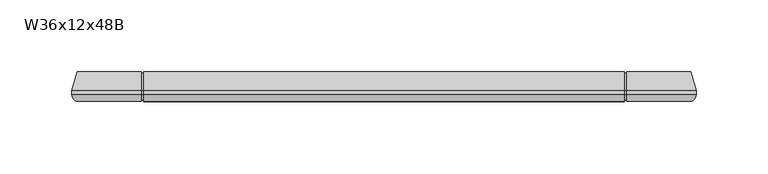
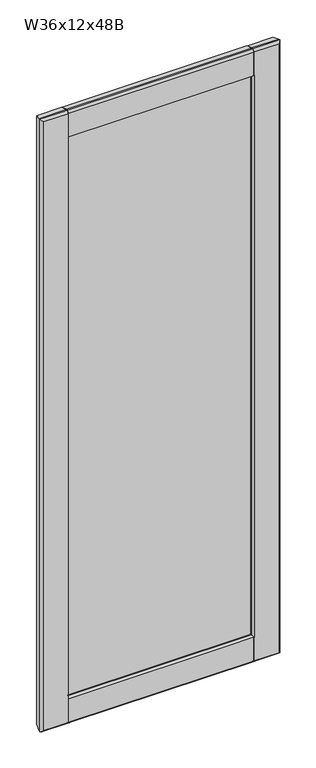
"""IFC4 building model written with IfcOpenShell, lengths in millimetres: furniture geometry, Cabinet-Wall-Merillat-Double_Door-Marlin : W36x12x48B."""

from ifc_helpers import new_model, si_unit, frame, origin, place, context, project, spatial, polyline, circle_curve, ellipse_curve, outline, extrude, source, transform, mapped, element, save
from ifc_brep_helpers import plane_surface, cylinder_surface, advanced_brep


def w36x12x48b_c809501e(model_context):
    return source(origin(), model_context, "Body", "SolidModel", [
        advanced_brep(
        [(541.0528392, -401.6121, 2108.2), (537.9563467, -406.0825, 2105.1035075), (537.9563467, -406.0825, 942.8964925), (541.0528392, -401.6121, 939.8), (541.0528392, -398.8435, 939.8), (541.0528392, -398.8435, 2108.2), (537.5476392, -385.7625, 943.3052), (537.5476392, -385.7625, 2104.6948), (492.8516765, -385.7625, 2059.9988372), (492.8516765, -385.7625, 988.0011628), (492.4815448, -386.55625, 988.3712945), (490.4003857, -391.01931, 990.4524535), (490.4003857, -391.01931, 2057.5475465), (492.4815448, -386.55625, 2059.6287055), (491.8001552, -393.2594093, 989.052684), (491.8001552, -393.2594093, 2058.947316), (506.1278392, -393.5095, 974.725), (506.1278392, -393.5095, 2073.275), (506.1278392, -398.3355, 974.725), (506.1278392, -398.3355, 2073.275), (491.8001552, -398.5855907, 989.052684), (491.8001552, -398.5855907, 2058.947316), (490.4003857, -400.82569, 990.4524535), (490.4003857, -400.82569, 2057.5475465), (492.4815448, -405.28875, 988.3712945), (492.848809, -406.0763508, 988.0040302), (492.8516765, -406.0825, 2059.9988372), (492.4815448, -405.28875, 2059.6287055), (492.848809, -406.0825, 942.8964925), (492.848809, -401.6121, 939.8), (110.7618317, -406.0825, 942.8964925), (107.6653392, -401.6121, 939.8), (155.8295579, -401.6121, 939.8), (155.8295579, -406.0825, 942.8964925), (491.261309, -401.6121, 939.8), (491.261309, -406.0825, 942.8964925), (157.4170579, -406.0825, 942.8964925), (157.4170579, -401.6121, 939.8), (492.848809, -398.8435, 939.8), (107.6653392, -398.8435, 939.8), (155.8295579, -398.8435, 939.8), (491.261309, -398.8435, 939.8), (157.4170579, -398.8435, 939.8), (492.848809, -385.7625, 943.3052), (111.1705392, -385.7625, 943.3052), (155.8295579, -385.7625, 943.3052), (491.261309, -385.7625, 943.3052), (157.4170579, -385.7625, 943.3052), (158.3177927, -391.01931, 990.4524535), (491.261309, -386.55625, 988.3712945), (491.261309, -385.7625, 988.0011628), (157.4170579, -385.7625, 988.0011628), (157.4170579, -386.55625, 988.3712945), (156.2366337, -386.55625, 988.3712945), (156.9180233, -393.2594093, 989.052684), (142.5903392, -393.5095, 974.725), (142.5903392, -398.3355, 974.725), (156.9180233, -398.5855907, 989.052684), (158.3177927, -400.82569, 990.4524535), (156.2366337, -405.28875, 988.3712945), (157.4170579, -405.28875, 988.3712945), (157.4170579, -406.0825, 988.0011628), (491.261309, -406.0825, 988.0011628), (491.261309, -405.28875, 988.3712945), (110.7618317, -406.0825, 2105.1035075), (107.6653392, -401.6121, 2108.2), (107.6653392, -398.8435, 2108.2), (111.1705392, -385.7625, 2104.6948), (155.866502, -385.7625, 988.0011628), (155.866502, -385.7625, 2059.9988372), (156.2366337, -386.55625, 2059.6287055), (158.3177927, -391.01931, 2057.5475465), (156.9180233, -393.2594093, 2058.947316), (142.5903392, -393.5095, 2073.275), (142.5903392, -398.3355, 2073.275), (156.9180233, -398.5855907, 2058.947316), (158.3177927, -400.82569, 2057.5475465), (156.2366337, -405.28875, 2059.6287055), (155.866502, -406.0825, 2059.9988372), (155.866502, -406.0825, 988.0011628), (155.8295579, -406.0825, 2105.1035075), (155.8295579, -401.6121, 2108.2), (492.848809, -401.6121, 2108.2), (492.848809, -406.0825, 2105.1035075), (157.4170579, -401.6121, 2108.2), (157.4170579, -406.0825, 2105.1035075), (491.261309, -406.0825, 2105.1035075), (491.261309, -401.6121, 2108.2), (155.8295579, -398.8435, 2108.2), (492.848809, -398.8435, 2108.2), (157.4170579, -398.8435, 2108.2), (491.261309, -398.8435, 2108.2), (155.8295579, -385.7625, 2104.6948), (492.848809, -385.7625, 2104.6948), (157.4170579, -385.7625, 2104.6948), (491.261309, -385.7625, 2104.6948), (157.4170579, -385.7625, 2059.9988372), (491.261309, -385.7625, 2059.9988372), (157.4170579, -386.55625, 2059.6287055), (491.261309, -386.55625, 2059.6287055), (491.261309, -405.28875, 2059.6287055), (491.261309, -406.0825, 2059.9988372), (157.4170579, -406.0825, 2059.9988372), (157.4170579, -405.28875, 2059.6287055), (157.4170579, -386.55625, 2104.0857412), (157.4170579, -398.9480037, 2107.40625), (157.4170579, -401.6121, 2107.40625), (157.4170579, -405.28875, 2104.9526052), (155.8295579, -405.28875, 2059.6287055), (155.8295579, -405.28875, 2104.9526052), (155.8295579, -401.6121, 2107.40625), (155.8295579, -398.9480037, 2107.40625), (155.8295579, -386.55625, 2104.0857412), (155.8295579, -386.55625, 2059.6287055), (492.848809, -386.55625, 2059.6287055), (492.848809, -386.55625, 2104.0857412), (492.848809, -398.9480037, 2107.40625), (492.848809, -401.6121, 2107.40625), (492.848809, -405.28875, 2104.9526052), (492.848809, -405.28875, 2059.6287055), (491.261309, -405.28875, 2104.9526052), (491.261309, -401.6121, 2107.40625), (491.261309, -398.9480037, 2107.40625), (491.261309, -386.55625, 2104.0857412), (492.848809, -405.28875, 988.3712945), (492.848809, -405.28875, 943.0473948), (492.848809, -401.6121, 940.59375), (492.848809, -398.9480037, 940.59375), (492.848809, -386.55625, 943.9142588), (492.848809, -386.55625, 988.3712945), (491.261309, -386.55625, 943.9142588), (491.261309, -398.9480037, 940.59375), (491.261309, -401.6121, 940.59375), (491.261309, -405.28875, 943.0473948), (157.4170579, -405.28875, 943.0473948), (157.4170579, -401.6121, 940.59375), (157.4170579, -398.9480037, 940.59375), (157.4170579, -386.55625, 943.9142588), (155.8295579, -405.28875, 988.3712945), (155.8295579, -386.55625, 988.3712945), (155.8295579, -386.55625, 943.9142588), (155.8295579, -398.9480037, 940.59375), (155.8295579, -401.6121, 940.59375), (155.8295579, -405.28875, 943.0473948)],
        [
            (0, 1, ellipse_curve(frame((536.2776392, -401.6121, 2103.4248), z_axis=(0.7071067811865475, 0.0, -0.7071067811865475), x_axis=(0.7071067811865474, 0.0, 0.7071067811865476)), 6.7531526, 4.7752)),
            (1, 2),
            (2, 3, ellipse_curve(frame((536.2776392, -401.6121, 944.5752), z_axis=(0.7071067811865475, 0.0, 0.7071067811865475), x_axis=(-0.7071067811865474, 0.0, 0.7071067811865476)), 6.7531526, 4.7752)),
            (3, 0),
            (3, 4),
            (4, 5),
            (5, 0),
            (4, 6),
            (6, 7),
            (7, 5),
            (8, 9),
            (9, 10),
            (10, 11),
            (11, 12),
            (12, 13),
            (13, 8),
            (11, 14, ellipse_curve(frame((491.8276392, -391.6848492, 989.0252), z_axis=(0.7071067811865475, 0.0, 0.7071067811865475), x_axis=(-0.7071067811865474, 0.0, 0.7071067811865476)), 2.2271035, 1.5748)),
            (14, 15),
            (15, 12, ellipse_curve(frame((491.8276392, -391.6848492, 2058.9748), z_axis=(0.7071067811865475, 0.0, -0.7071067811865475), x_axis=(0.7071067811865474, 0.0, 0.7071067811865476)), 2.2271035, 1.5748)),
            (14, 16),
            (16, 17),
            (17, 15),
            (16, 18),
            (18, 19),
            (19, 17),
            (18, 20),
            (20, 21),
            (21, 19),
            (20, 22, ellipse_curve(frame((491.8276392, -400.1601508, 989.0252), z_axis=(0.7071067811865475, 0.0, 0.7071067811865475), x_axis=(-0.7071067811865474, 0.0, 0.7071067811865476)), 2.2271035, 1.5748)),
            (22, 23),
            (23, 21, ellipse_curve(frame((491.8276392, -400.1601508, 2058.9748), z_axis=(0.7071067811865475, 0.0, -0.7071067811865475), x_axis=(0.7071067811865474, 0.0, 0.7071067811865476)), 2.2271035, 1.5748)),
            (22, 24),
            (24, 25),
            (25, 26),
            (26, 27),
            (27, 23),
            (2, 28),
            (28, 29, circle_curve(frame((492.848809, -401.6121, 944.5752), z_axis=(1.0, 0.0, 0.0), x_axis=(0.0, 1.0, 0.0)), 4.7752)),
            (29, 3),
            (30, 31, ellipse_curve(frame((112.4405392, -401.6121, 944.5752), z_axis=(0.7071067811865475, 0.0, -0.7071067811865475), x_axis=(0.7071067811865476, 0.0, 0.7071067811865474)), 6.7531526, 4.7752)),
            (31, 32),
            (32, 33, circle_curve(frame((155.8295579, -401.6121, 944.5752), z_axis=(-1.0, 0.0, 0.0), x_axis=(0.0, 1.0, 0.0)), 4.7752)),
            (33, 30),
            (34, 35, circle_curve(frame((491.261309, -401.6121, 944.5752), z_axis=(-1.0, 0.0, 0.0), x_axis=(0.0, 1.0, 0.0)), 4.7752)),
            (35, 36),
            (36, 37, circle_curve(frame((157.4170579, -401.6121, 944.5752), z_axis=(1.0, 0.0, 0.0), x_axis=(0.0, 1.0, 0.0)), 4.7752)),
            (37, 34),
            (29, 38),
            (38, 4),
            (31, 39),
            (39, 40),
            (40, 32),
            (41, 34),
            (37, 42),
            (42, 41),
            (38, 43),
            (43, 6),
            (39, 44),
            (44, 45),
            (45, 40),
            (46, 41),
            (42, 47),
            (47, 46),
            (48, 11),
            (10, 49),
            (49, 50),
            (50, 51),
            (51, 52),
            (52, 53),
            (53, 48),
            (48, 54, ellipse_curve(frame((156.8905392, -391.6848492, 989.0252), z_axis=(0.7071067811865475, 0.0, -0.7071067811865475), x_axis=(0.7071067811865476, 0.0, 0.7071067811865474)), 2.2271035, 1.5748)),
            (54, 14),
            (54, 55),
            (55, 16),
            (55, 56),
            (56, 18),
            (56, 57),
            (57, 20),
            (57, 58, ellipse_curve(frame((156.8905392, -400.1601508, 989.0252), z_axis=(0.7071067811865475, 0.0, -0.7071067811865475), x_axis=(0.7071067811865476, 0.0, 0.7071067811865474)), 2.2271035, 1.5748)),
            (58, 22),
            (58, 59),
            (59, 60),
            (60, 61),
            (61, 62),
            (62, 63),
            (63, 24),
            (30, 64),
            (64, 65, ellipse_curve(frame((112.4405392, -401.6121, 2103.4248), z_axis=(-0.7071067811865475, 0.0, -0.7071067811865475), x_axis=(0.7071067811865474, 0.0, -0.7071067811865476)), 6.7531526, 4.7752)),
            (65, 31),
            (65, 66),
            (66, 39),
            (66, 67),
            (67, 44),
            (68, 69),
            (69, 70),
            (70, 71),
            (71, 48),
            (53, 68),
            (71, 72, ellipse_curve(frame((156.8905392, -391.6848492, 2058.9748), z_axis=(-0.7071067811865475, 0.0, -0.7071067811865475), x_axis=(0.7071067811865474, 0.0, -0.7071067811865476)), 2.2271035, 1.5748)),
            (72, 54),
            (72, 73),
            (73, 55),
            (73, 74),
            (74, 56),
            (74, 75),
            (75, 57),
            (75, 76, ellipse_curve(frame((156.8905392, -400.1601508, 2058.9748), z_axis=(-0.7071067811865475, 0.0, -0.7071067811865475), x_axis=(0.7071067811865474, 0.0, -0.7071067811865476)), 2.2271035, 1.5748)),
            (76, 58),
            (76, 77),
            (77, 78),
            (78, 79),
            (79, 59),
            (64, 80),
            (80, 81, circle_curve(frame((155.8295579, -401.6121, 2103.4248), z_axis=(-1.0, 0.0, 0.0), x_axis=(0.0, 1.0, 0.0)), 4.7752)),
            (81, 65),
            (0, 82),
            (82, 83, circle_curve(frame((492.848809, -401.6121, 2103.4248), z_axis=(1.0, 0.0, 0.0), x_axis=(0.0, 1.0, 0.0)), 4.7752)),
            (83, 1),
            (84, 85, circle_curve(frame((157.4170579, -401.6121, 2103.4248), z_axis=(1.0, 0.0, 0.0), x_axis=(0.0, 1.0, 0.0)), 4.7752)),
            (85, 86),
            (86, 87, circle_curve(frame((491.261309, -401.6121, 2103.4248), z_axis=(-1.0, 0.0, 0.0), x_axis=(0.0, 1.0, 0.0)), 4.7752)),
            (87, 84),
            (81, 88),
            (88, 66),
            (5, 89),
            (89, 82),
            (90, 84),
            (87, 91),
            (91, 90),
            (88, 92),
            (92, 67),
            (7, 93),
            (93, 89),
            (94, 90),
            (91, 95),
            (95, 94),
            (92, 69),
            (68, 45),
            (50, 46),
            (47, 51),
            (43, 9),
            (8, 93),
            (96, 94),
            (95, 97),
            (97, 96),
            (12, 71),
            (70, 98),
            (98, 96),
            (97, 99),
            (99, 13),
            (15, 72),
            (17, 73),
            (19, 74),
            (21, 75),
            (23, 76),
            (27, 100),
            (100, 101),
            (101, 102),
            (102, 103),
            (103, 77),
            (83, 26),
            (25, 28),
            (33, 79),
            (78, 80),
            (35, 62),
            (61, 36),
            (85, 102),
            (101, 86),
            (98, 104),
            (104, 105),
            (105, 106),
            (106, 107, circle_curve(frame((157.4170579, -401.6121, 2103.4248), z_axis=(1.0, 0.0, 0.0), x_axis=(0.0, 0.0, 1.0)), 3.98145)),
            (107, 103),
            (78, 108),
            (108, 109),
            (109, 110, circle_curve(frame((155.8295579, -401.6121, 2103.4248), z_axis=(-1.0, 0.0, 0.0), x_axis=(0.0, 0.0, 1.0)), 3.98145)),
            (110, 111),
            (111, 112),
            (112, 113),
            (113, 69),
            (77, 108),
            (107, 109),
            (106, 110),
            (105, 111),
            (104, 112),
            (70, 113),
            (8, 114),
            (114, 115),
            (115, 116),
            (116, 117),
            (117, 118, circle_curve(frame((492.848809, -401.6121, 2103.4248), z_axis=(1.0, 0.0, 0.0), x_axis=(0.0, 0.0, 1.0)), 3.98145)),
            (118, 119),
            (119, 26),
            (100, 120),
            (120, 121, circle_curve(frame((491.261309, -401.6121, 2103.4248), z_axis=(-1.0, 0.0, 0.0), x_axis=(0.0, 0.0, 1.0)), 3.98145)),
            (121, 122),
            (122, 123),
            (123, 99),
            (119, 27),
            (118, 120),
            (117, 121),
            (116, 122),
            (115, 123),
            (114, 13),
            (25, 124),
            (124, 125),
            (125, 126, circle_curve(frame((492.848809, -401.6121, 944.5752), z_axis=(1.0, 0.0, 0.0), x_axis=(0.0, 0.0, 1.0)), 3.98145)),
            (126, 127),
            (127, 128),
            (128, 129),
            (129, 9),
            (49, 130),
            (130, 131),
            (131, 132),
            (132, 133, circle_curve(frame((491.261309, -401.6121, 944.5752), z_axis=(-1.0, 0.0, 0.0), x_axis=(0.0, 0.0, 1.0)), 3.98145)),
            (133, 63),
            (129, 10),
            (128, 130),
            (127, 131),
            (126, 132),
            (125, 133),
            (124, 24),
            (60, 134),
            (134, 135, circle_curve(frame((157.4170579, -401.6121, 944.5752), z_axis=(1.0, 0.0, 0.0), x_axis=(0.0, 0.0, 1.0)), 3.98145)),
            (135, 136),
            (136, 137),
            (137, 52),
            (138, 79),
            (68, 139),
            (139, 140),
            (140, 141),
            (141, 142),
            (142, 143, circle_curve(frame((155.8295579, -401.6121, 944.5752), z_axis=(-1.0, 0.0, 0.0), x_axis=(0.0, 0.0, 1.0)), 3.98145)),
            (143, 138),
            (138, 59),
            (53, 139),
            (137, 140),
            (136, 141),
            (135, 142),
            (134, 143),
        ],
        [
            cylinder_surface(frame((536.2776392, -401.6121, 2108.2), z_axis=(0.0, 0.0, 1.0), x_axis=(0.0, 1.0, 0.0)), 4.7752),
            plane_surface(frame((541.0528392, -401.6121, 2108.2), z_axis=(1.0, 0.0, 0.0), x_axis=(0.0, 0.0, -1.0))),
            plane_surface(frame((541.0528392, -398.8435, 2108.2), z_axis=(0.9659229350723619, 0.25882983502910506, 0.0), x_axis=(0.0, 0.0, -1.0))),
            plane_surface(frame((492.8516765, -385.7625, 2059.9988372), z_axis=(-0.9063077870366099, 0.4226182617407856, 0.0), x_axis=(0.0, 0.0, -1.0))),
            cylinder_surface(frame((491.8276392, -391.6848492, 2108.2), z_axis=(0.0, 0.0, 1.0000000000000002), x_axis=(-0.01745240643729364, -0.9998476951563912, 0.0)), 1.5748),
            plane_surface(frame((491.8001552, -393.2594093, 2058.947316), z_axis=(-0.017452406437322144, -0.9998476951563906, 0.0), x_axis=(0.0, 0.0, -1.0))),
            plane_surface(frame((506.1278392, -393.5095, 2073.275), z_axis=(-1.0, 0.0, 0.0), x_axis=(0.0, 0.0, -1.0))),
            plane_surface(frame((506.1278392, -398.3355, 2073.275), z_axis=(-0.01745240643727848, 0.9998476951563914, 0.0), x_axis=(0.0, 0.0, -1.0))),
            cylinder_surface(frame((491.8276392, -400.1601508, 2108.2), z_axis=(0.0, 0.0, 1.0000000000000002), x_axis=(-0.9063077870367326, -0.42261826174052236, 0.0)), 1.5748),
            plane_surface(frame((490.4003857, -400.82569, 2057.5475465), z_axis=(-0.9063077870366333, -0.4226182617407352, 0.0), x_axis=(0.0, 0.0, -1.0))),
            cylinder_surface(frame((541.0528392, -401.6121, 944.5752), z_axis=(1.0, 0.0, 0.0), x_axis=(0.0, 1.0, 0.0)), 4.7752),
            plane_surface(frame((541.0528392, -401.6121, 939.8), z_axis=(0.0, 0.0, -1.0), x_axis=(-1.0, 0.0, 0.0))),
            plane_surface(frame((541.0528392, -398.8435, 939.8), z_axis=(0.0, 0.2588298350291095, -0.9659229350723607), x_axis=(-1.0, 0.0, 0.0))),
            plane_surface(frame((492.8516765, -385.7625, 988.0011628), z_axis=(0.0, 0.42261826174078143, 0.9063077870366119), x_axis=(-1.0, 0.0, 0.0))),
            cylinder_surface(frame((541.0528392, -391.6848492, 989.0252), z_axis=(1.0000000000000002, 0.0, 0.0), x_axis=(0.0, -0.9998476951563913, 0.017452406437289025)), 1.5748),
            plane_surface(frame((491.8001552, -393.2594093, 989.052684), z_axis=(0.0, -0.9998476951563907, 0.01745240643731753), x_axis=(-1.0, 0.0, 0.0))),
            plane_surface(frame((506.1278392, -393.5095, 974.725), z_axis=(0.0, 0.0, 1.0), x_axis=(-1.0, 0.0, 0.0))),
            plane_surface(frame((506.1278392, -398.3355, 974.725), z_axis=(0.0, 0.9998476951563913, 0.017452406437283095), x_axis=(-1.0, 0.0, 0.0))),
            cylinder_surface(frame((541.0528392, -400.1601508, 989.0252), z_axis=(1.0000000000000002, 0.0, 0.0), x_axis=(0.0, -0.4226182617405265, 0.9063077870367306)), 1.5748),
            plane_surface(frame((490.4003857, -400.82569, 990.4524535), z_axis=(0.0, -0.4226182617407394, 0.9063077870366314), x_axis=(-1.0, 0.0, 0.0))),
            cylinder_surface(frame((112.4405392, -401.6121, 939.8), z_axis=(0.0, 0.0, -1.0), x_axis=(0.0, 1.0, 0.0)), 4.7752),
            plane_surface(frame((107.6653392, -401.6121, 939.8), z_axis=(-1.0, 0.0, 0.0), x_axis=(0.0, 0.0, 1.0))),
            plane_surface(frame((107.6653392, -398.8435, 939.8), z_axis=(-0.9659229350723619, 0.25882983502910506, 0.0), x_axis=(0.0, 0.0, 1.0))),
            plane_surface(frame((155.866502, -385.7625, 988.0011628), z_axis=(0.9063077870366099, 0.4226182617407856, 0.0), x_axis=(0.0, 0.0, 1.0))),
            cylinder_surface(frame((156.8905392, -391.6848492, 939.8), z_axis=(0.0, 0.0, -1.0000000000000002), x_axis=(0.01745240643729364, -0.9998476951563912, 0.0)), 1.5748),
            plane_surface(frame((156.9180233, -393.2594093, 989.052684), z_axis=(0.017452406437322144, -0.9998476951563906, 0.0), x_axis=(0.0, 0.0, 1.0))),
            plane_surface(frame((142.5903392, -393.5095, 974.725), z_axis=(1.0, 0.0, 0.0), x_axis=(0.0, 0.0, 1.0))),
            plane_surface(frame((142.5903392, -398.3355, 974.725), z_axis=(0.01745240643727848, 0.9998476951563914, 0.0), x_axis=(0.0, 0.0, 1.0))),
            cylinder_surface(frame((156.8905392, -400.1601508, 939.8), z_axis=(0.0, 0.0, -1.0000000000000002), x_axis=(0.9063077870367326, -0.42261826174052236, 0.0)), 1.5748),
            plane_surface(frame((158.3177927, -400.82569, 990.4524535), z_axis=(0.9063077870366333, -0.4226182617407352, 0.0), x_axis=(0.0, 0.0, 1.0))),
            cylinder_surface(frame((107.6653392, -401.6121, 2103.4248), z_axis=(-1.0, 0.0, 0.0), x_axis=(0.0, 1.0, 0.0)), 4.7752),
            plane_surface(frame((107.6653392, -401.6121, 2108.2), z_axis=(0.0, 0.0, 1.0), x_axis=(1.0, 0.0, 0.0))),
            plane_surface(frame((107.6653392, -398.8435, 2108.2), z_axis=(0.0, 0.2588298350291006, 0.9659229350723632), x_axis=(1.0, 0.0, 0.0))),
            plane_surface(frame((111.1705392, -385.7625, 2104.6948), z_axis=(0.0, 1.0, 0.0), x_axis=(1.0, 0.0, 0.0))),
            plane_surface(frame((155.866502, -385.7625, 2059.9988372), z_axis=(0.0, 0.42261826174078976, -0.9063077870366079), x_axis=(1.0, 0.0, 0.0))),
            cylinder_surface(frame((107.6653392, -391.6848492, 2058.9748), z_axis=(-1.0000000000000002, 0.0, 0.0), x_axis=(0.0, -0.999847695156391, -0.017452406437298253)), 1.5748),
            plane_surface(frame((156.9180233, -393.2594093, 2058.947316), z_axis=(0.0, -0.9998476951563905, -0.01745240643732676), x_axis=(1.0, 0.0, 0.0))),
            plane_surface(frame((142.5903392, -393.5095, 2073.275), z_axis=(0.0, 0.0, -1.0), x_axis=(1.0, 0.0, 0.0))),
            plane_surface(frame((142.5903392, -398.3355, 2073.275), z_axis=(0.0, 0.9998476951563915, -0.017452406437273867), x_axis=(1.0, 0.0, 0.0))),
            cylinder_surface(frame((107.6653392, -400.1601508, 2058.9748), z_axis=(-1.0000000000000002, 0.0, 0.0), x_axis=(0.0, -0.4226182617405182, -0.9063077870367346)), 1.5748),
            plane_surface(frame((158.3177927, -400.82569, 2057.5475465), z_axis=(0.0, -0.422618261740731, -0.9063077870366353), x_axis=(1.0, 0.0, 0.0))),
            plane_surface(frame((155.866502, -406.0825, 2059.9988372), z_axis=(0.0, -1.0, 0.0), x_axis=(1.0, 0.0, 0.0))),
            plane_surface(frame((157.4170579, -406.0825, 2059.9988372), z_axis=(-1.0000000000000002, 0.0, 0.0), x_axis=(0.0, 0.906307787036639, -0.4226182617407233))),
            plane_surface(frame((155.8295579, -406.0825, 2059.9988372), z_axis=(1.0000000000000002, 0.0, 0.0), x_axis=(0.0, -0.906307787036639, 0.4226182617407233))),
            plane_surface(frame((157.4170579, -406.0825, 2059.9988372), z_axis=(0.0, 0.4226182617407233, 0.906307787036639), x_axis=(-1.0, 0.0, 0.0))),
            plane_surface(frame((157.4170579, -405.28875, 2059.6287055), z_axis=(0.0, -1.0, 0.0), x_axis=(-1.0, 0.0, 0.0))),
            cylinder_surface(frame((155.8295579, -401.6121, 2103.4248), z_axis=(-1.0, 0.0, 0.0), x_axis=(0.0, 0.0, 1.0)), 3.98145),
            plane_surface(frame((157.4170579, -401.6121, 2107.40625), z_axis=(0.0, 0.0, 1.0), x_axis=(-1.0, 0.0, 0.0))),
            plane_surface(frame((157.4170579, -398.9480037, 2107.40625), z_axis=(0.0, 0.25882983502917667, 0.9659229350723427), x_axis=(-1.0, 0.0, 0.0))),
            plane_surface(frame((157.4170579, -386.55625, 2104.0857412), z_axis=(0.0, 1.0, 0.0), x_axis=(-1.0, 0.0, 0.0))),
            plane_surface(frame((157.4170579, -386.55625, 2059.6287055), z_axis=(0.0, -0.4226182617408151, 0.906307787036596), x_axis=(-1.0, 0.0, 0.0))),
            plane_surface(frame((492.848809, -406.0825, 2059.9988372), z_axis=(-1.0000000000000002, 0.0, 0.0), x_axis=(0.0, 0.9063077870366527, -0.4226182617406937))),
            plane_surface(frame((491.261309, -406.0825, 2059.9988372), z_axis=(1.0000000000000002, 0.0, 0.0), x_axis=(0.0, -0.9063077870366527, 0.4226182617406937))),
            plane_surface(frame((492.848809, -406.0825, 2059.9988372), z_axis=(0.0, 0.4226182617406937, 0.9063077870366527), x_axis=(-1.0, 0.0, 0.0))),
            plane_surface(frame((492.848809, -405.28875, 2059.6287055), z_axis=(0.0, -1.0, 0.0), x_axis=(-1.0, 0.0, 0.0))),
            cylinder_surface(frame((491.261309, -401.6121, 2103.4248), z_axis=(-1.0, 0.0, 0.0), x_axis=(0.0, 0.0, 1.0)), 3.98145),
            plane_surface(frame((492.848809, -401.6121, 2107.40625), z_axis=(0.0, 0.0, 1.0), x_axis=(-1.0, 0.0, 0.0))),
            plane_surface(frame((492.848809, -398.9480037, 2107.40625), z_axis=(0.0, 0.25882983502917556, 0.9659229350723431), x_axis=(-1.0, 0.0, 0.0))),
            plane_surface(frame((492.848809, -386.55625, 2104.0857412), z_axis=(0.0, 1.0, 0.0), x_axis=(-1.0, 0.0, 0.0))),
            plane_surface(frame((492.848809, -386.55625, 2059.6287055), z_axis=(0.0, -0.4226182617408452, 0.906307787036582), x_axis=(-1.0, 0.0, 0.0))),
            plane_surface(frame((492.848809, -401.6121, 949.3504), z_axis=(-1.0, 0.0, 0.0), x_axis=(0.0, -1.0, 0.0))),
            plane_surface(frame((491.261309, -401.6121, 949.3504), z_axis=(1.0, 0.0, 0.0), x_axis=(0.0, 1.0, 0.0))),
            plane_surface(frame((492.848809, -385.7625, 988.0011628), z_axis=(0.0, -0.4226182617407559, -0.9063077870366237), x_axis=(-1.0, 0.0, 0.0))),
            plane_surface(frame((492.848809, -386.55625, 988.3712945), z_axis=(0.0, 1.0, 0.0), x_axis=(-1.0, 0.0, 0.0))),
            plane_surface(frame((492.848809, -386.55625, 943.9142588), z_axis=(0.0, 0.2588298350294462, -0.9659229350722706), x_axis=(-1.0, 0.0, 0.0))),
            plane_surface(frame((492.848809, -398.9480037, 940.59375), z_axis=(0.0, 0.0, -1.0), x_axis=(-1.0, 0.0, 0.0))),
            cylinder_surface(frame((491.261309, -401.6121, 944.5752), z_axis=(-1.0, 0.0, 0.0), x_axis=(0.0, 0.0, 1.0)), 3.98145),
            plane_surface(frame((492.848809, -405.28875, 943.0473948), z_axis=(0.0, -1.0, 0.0), x_axis=(-1.0, 0.0, 0.0))),
            plane_surface(frame((492.848809, -405.28875, 988.3712945), z_axis=(0.0, 0.4226182617407407, -0.9063077870366308), x_axis=(-1.0, 0.0, 0.0))),
            plane_surface(frame((157.4170579, -405.28875, 988.3712945), z_axis=(-1.0000000000000002, 0.0, 0.0), x_axis=(0.0, -0.906307787036642, -0.42261826174071665))),
            plane_surface(frame((155.8295579, -405.28875, 988.3712945), z_axis=(1.0000000000000002, 0.0, 0.0), x_axis=(0.0, 0.906307787036642, 0.42261826174071665))),
            plane_surface(frame((157.4170579, -405.28875, 988.3712945), z_axis=(0.0, 0.42261826174071665, -0.906307787036642), x_axis=(-1.0, 0.0, 0.0))),
            plane_surface(frame((157.4170579, -385.7625, 988.0011628), z_axis=(0.0, -0.42261826174079165, -0.9063077870366071), x_axis=(-1.0, 0.0, 0.0))),
            plane_surface(frame((157.4170579, -386.55625, 988.3712945), z_axis=(0.0, 1.0, 0.0), x_axis=(-1.0, 0.0, 0.0))),
            plane_surface(frame((157.4170579, -386.55625, 943.9142588), z_axis=(0.0, 0.2588298350294473, -0.9659229350722702), x_axis=(-1.0, 0.0, 0.0))),
            plane_surface(frame((157.4170579, -398.9480037, 940.59375), z_axis=(0.0, 0.0, -1.0), x_axis=(-1.0, 0.0, 0.0))),
            cylinder_surface(frame((155.8295579, -401.6121, 944.5752), z_axis=(-1.0, 0.0, 0.0), x_axis=(0.0, 0.0, 1.0)), 3.98145),
            plane_surface(frame((157.4170579, -405.28875, 943.0473948), z_axis=(0.0, -1.0, 0.0), x_axis=(-1.0, 0.0, 0.0))),
        ],
        [
            (0, [[1, 2, 3, 4]]),
            (1, [[-4, 5, 6, 7]]),
            (2, [[-6, 8, 9, 10]]),
            (3, [[11, 12, 13, 14, 15, 16]]),
            (4, [[-14, 17, 18, 19]]),
            (5, [[-18, 20, 21, 22]]),
            (6, [[-21, 23, 24, 25]]),
            (7, [[-24, 26, 27, 28]]),
            (8, [[-27, 29, 30, 31]]),
            (9, [[-30, 32, 33, 34, 35, 36]]),
            (10, [[-3, 37, 38, 39]]),
            (10, [[40, 41, 42, 43]]),
            (10, [[44, 45, 46, 47]]),
            (11, [[-5, -39, 48, 49]]),
            (11, [[50, 51, 52, -41]]),
            (11, [[53, -47, 54, 55]]),
            (12, [[-8, -49, 56, 57]]),
            (12, [[58, 59, 60, -51]]),
            (12, [[61, -55, 62, 63]]),
            (13, [[64, -13, 65, 66, 67, 68, 69, 70]]),
            (14, [[-17, -64, 71, 72]]),
            (15, [[-20, -72, 73, 74]]),
            (16, [[-23, -74, 75, 76]]),
            (17, [[-26, -76, 77, 78]]),
            (18, [[-29, -78, 79, 80]]),
            (19, [[-80, 81, 82, 83, 84, 85, 86, -32]]),
            (20, [[-40, 87, 88, 89]]),
            (21, [[-50, -89, 90, 91]]),
            (22, [[-58, -91, 92, 93]]),
            (23, [[94, 95, 96, 97, -70, 98]]),
            (24, [[-71, -97, 99, 100]]),
            (25, [[-73, -100, 101, 102]]),
            (26, [[-75, -102, 103, 104]]),
            (27, [[-77, -104, 105, 106]]),
            (28, [[-79, -106, 107, 108]]),
            (29, [[-108, 109, 110, 111, 112, -81]]),
            (30, [[-88, 113, 114, 115]]),
            (30, [[-1, 116, 117, 118]]),
            (30, [[119, 120, 121, 122]]),
            (31, [[-90, -115, 123, 124]]),
            (31, [[-7, 125, 126, -116]]),
            (31, [[127, -122, 128, 129]]),
            (32, [[-92, -124, 130, 131]]),
            (32, [[-10, 132, 133, -125]]),
            (32, [[134, -129, 135, 136]]),
            (33, [[-93, -131, 137, -94, 138, -59]]),
            (33, [[139, -63, 140, -67]]),
            (33, [[-9, -57, 141, -11, 142, -132]]),
            (33, [[143, -136, 144, 145]]),
            (34, [[146, -96, 147, 148, -145, 149, 150, -15]]),
            (35, [[-19, 151, -99, -146]]),
            (36, [[-22, 152, -101, -151]]),
            (37, [[-25, 153, -103, -152]]),
            (38, [[-28, 154, -105, -153]]),
            (39, [[-31, 155, -107, -154]]),
            (40, [[-155, -36, 156, 157, 158, 159, 160, -109]]),
            (41, [[-2, -118, 161, -34, 162, -37]]),
            (41, [[-87, -43, 163, -111, 164, -113]]),
            (41, [[165, -84, 166, -45]]),
            (41, [[167, -158, 168, -120]]),
            (42, [[169, 170, 171, 172, 173, -159, -167, -119, -127, -134, -143, -148]]),
            (43, [[174, 175, 176, 177, 178, 179, 180, -137, -130, -123, -114, -164]]),
            (44, [[-174, -110, 181]]),
            (45, [[-173, 182, -175, -181, -160]]),
            (46, [[-172, 183, -176, -182]]),
            (47, [[-171, 184, -177, -183]]),
            (48, [[-170, 185, -178, -184]]),
            (49, [[-169, -147, 186, -179, -185]]),
            (50, [[-180, -186, -95]]),
            (51, [[187, 188, 189, 190, 191, 192, 193, -161, -117, -126, -133, -142]]),
            (52, [[194, 195, 196, 197, 198, -149, -144, -135, -128, -121, -168, -157]]),
            (53, [[-193, 199, -35]]),
            (54, [[-192, 200, -194, -156, -199]]),
            (55, [[-191, 201, -195, -200]]),
            (56, [[-190, 202, -196, -201]]),
            (57, [[-189, 203, -197, -202]]),
            (58, [[-188, 204, -150, -198, -203]]),
            (59, [[-187, -16, -204]]),
            (60, [[205, 206, 207, 208, 209, 210, 211, -141, -56, -48, -38, -162]]),
            (61, [[212, 213, 214, 215, 216, -85, -165, -44, -53, -61, -139, -66]]),
            (62, [[-211, 217, -12]]),
            (63, [[-210, 218, -212, -65, -217]]),
            (64, [[-209, 219, -213, -218]]),
            (65, [[-208, 220, -214, -219]]),
            (66, [[-207, 221, -215, -220]]),
            (67, [[-206, 222, -86, -216, -221]]),
            (68, [[-205, -33, -222]]),
            (69, [[223, 224, 225, 226, 227, -68, -140, -62, -54, -46, -166, -83]]),
            (70, [[228, -163, -42, -52, -60, -138, 229, 230, 231, 232, 233, 234]]),
            (71, [[-228, 235, -112]]),
            (72, [[-229, -98, 236]]),
            (73, [[-227, 237, -230, -236, -69]]),
            (74, [[-226, 238, -231, -237]]),
            (75, [[-225, 239, -232, -238]]),
            (76, [[-224, 240, -233, -239]]),
            (77, [[-223, -82, -235, -234, -240]]),
        ],
    ),
        extrude(outline(polyline([(142.5903392, -398.3355), (142.5903392, -393.5095), (506.1278392, -393.5095), (506.1278392, -398.3355), (142.5903392, -398.3355)])), frame((0.0, 0.0, 974.725), z_axis=(0.0, 0.0, 1.0), x_axis=(1.0, 0.0, 0.0)), (0.0, 0.0, 1.0), 1098.55),
    ])


if __name__ == "__main__":
    model = new_model("IFC4")
    model_context = context("Model", 3, world=origin())
    ifc_project = project(units=[si_unit("LENGTHUNIT", "METRE", prefix="MILLI")], contexts=[model_context])
    site = spatial("IfcSite", under=ifc_project)
    building = spatial("IfcBuilding", under=site)
    placement = place(None, origin())
    w36x12x48b_shape = w36x12x48b_c809501e(model_context)
    element("IfcFurniture", 1, ObjectType="Cabinet-Wall-Merillat-Double_Door-Marlin : W36x12x48B", at=placement, inside=building, context=model_context, shape_type="MappedRepresentation", body=[
        mapped(w36x12x48b_shape, transform((0.0, 0.0, 0.0), x_axis=(1.0, 0.0, 0.0), y_axis=(0.0, 1.0, 0.0), z_axis=(0.0, 0.0, 1.0))),
    ])
    save(model, "model.ifc")

# Revit data of these elements
# Type "Cabinet-Wall-Merillat-Double_Door-Marlin : W36x12x48B"
#   URL = "https://www.merillat.com/"
#   Product Page URL = "https://www.merillat.com/our-products/"
#   Product Line = "Express"
#   Product Group = "Wall Cabinet"
#   Product Documentation Link = "http://merillatbusiness.com/wp-content/uploads/2014/07/Merillat_Classic_Catalog.pdf"
#   Model = "W3642B"
#   Manufacturer = "Merillat"
#   Height Note = "Actual Height of 21 inches Cabinet is 20 1/2 inches"
#   Glass Door Note = "Glass Cabinet doors are only available in specific sizes. Please refer to the catalog for this information before requesting a glass size."
#   Finish = "Wood"
#   Description = "Wall 3642 Butt Door"
#   Construction Type = "Wall Cabinet"
#   Cabinet Construction Note = "Cabinets with B suffix have BUTT doors without a center frame stile:"
#   Assembly Code = "C1030410"
#   Spacing = 0' - 1"
#   Shelving Height = 0' - 11 1/4"
#   Door Spacing = 0' - 0 1/8"
#   Cabinet Door Width = 1' - 5 1/16"
#   Cabinet Door Height = 3' - 10"
#   Depth = 1' - 0"
#   Height = 4' - 0"
#   Top Of Cabinet = 7' - 0"
#   Width = 3' - 0"
#   COBie.Type = no
#   Top and Bottom Visibility = yes
#   Partial Overlay Butt = yes
#   Partial Overlay = no
#   Number of Shelves Greater than one = 3
#   Number of Shelves = 3
#   Middle Shelf = yes
#   Full Overlay Butt = no
#   Full Overlay = no
#   Elevation Swing Line = yes
#   Door Drawer Material = Wood - Merillat - Pecan(1)
#   Cabinet Material = Wood - Merillat - Pecan(1)
#   Cabinet Door Style = element 806847
# Element 1 (IfcFurniture, "Cabinet-Wall-Merillat-Double_Door-Marlin : W36x12x48B")
#   Materials on its faces: "Wood - Merillat - Pecan(1)"
# Materials
#   "Wood - Merillat - Pecan(1)": class "Wood", colour RGB 108 67 43, transparency 0, Cost = 0
